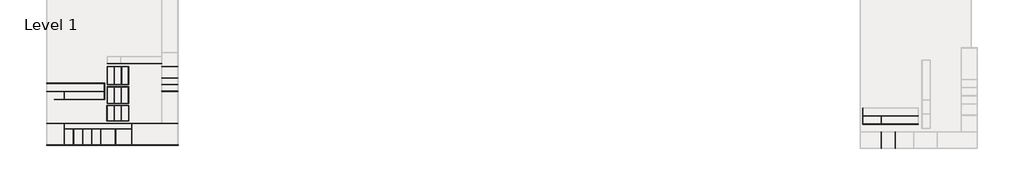
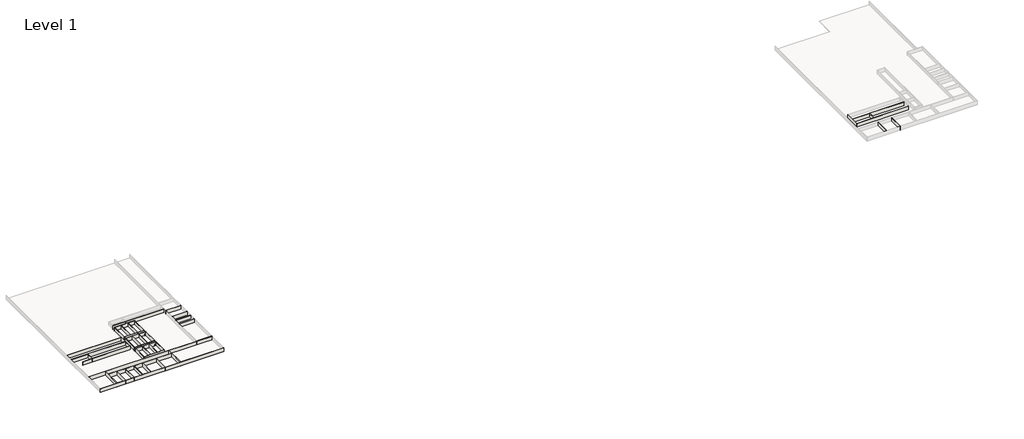
# One storey, part 1 of 4: 45 walls, 12 doors.
# Revit data of these elements (continued)
# Room at (1606634.071, 111947.24) mm, phase "New Construction", upper level "Level 1", upper offset 10.00 ft, lower offset 0.00 ft (continued)
#   Name = "STORAGE"
# Room at (1599894.048, 116775.918) mm, phase "New Construction", upper level "Level 1", upper offset 10.00 ft, lower offset 0.00 ft
#   Number = "64"
#   Name = "Room"
# Room at (1649995.832, 63944.956) mm, phase "New Construction", upper level "Level 1", upper offset 10.00 ft, lower offset 0.00 ft
#   Number = "65"
#   Name = "CLASSROOM"
# Room, not placed, phase "New Construction", upper offset 0.00 ft, lower offset 0.00 ft
#   Number = "165"
#   Name = "RETAIL"
# Room, not placed, phase "New Construction", upper offset 0.00 ft, lower offset 0.00 ft
#   Number = "166"
#   Name = "KITCHEN/CONCESSIONS"
# Room, not placed, phase "New Construction", upper offset 0.00 ft, lower offset 0.00 ft
#   Number = "167"
#   Name = "RETAIL"
# Room, not placed, phase "New Construction", upper offset 0.00 ft, lower offset 0.00 ft
#   Number = "168"
#   Name = "RETAIL"
# Room, not placed, phase "New Construction", upper offset 0.00 ft, lower offset 0.00 ft
#   Number = "169"
#   Name = "XCEL ENTRANCE/LOBBY"
# Room, not placed, phase "New Construction", upper offset 0.00 ft, lower offset 0.00 ft
#   Number = "170"
#   Name = "CLINIC"
# Room, not placed, phase "New Construction", upper offset 0.00 ft, lower offset 0.00 ft
#   Number = "171"
#   Name = "Clinic"
# Room, not placed, phase "New Construction", upper offset 0.00 ft, lower offset 0.00 ft
#   Number = "172"
#   Name = "Room"
# Room, not placed, phase "New Construction", upper offset 0.00 ft, lower offset 0.00 ft
#   Number = "173"
#   Name = "RETAIL"
# Room, not placed, phase "New Construction", upper offset 0.00 ft, lower offset 0.00 ft
#   Number = "174"
#   Name = "RETAIL"
# Room, not placed, phase "New Construction", upper offset 0.00 ft, lower offset 0.00 ft
#   Number = "175"
#   Name = "RETAIL"
# Room, not placed, phase "New Construction", upper offset 0.00 ft, lower offset 0.00 ft
#   Number = "176"
#   Name = "RETAIL"
# Room, not placed, phase "New Construction", upper offset 0.00 ft, lower offset 0.00 ft
#   Number = "177"
#   Name = "Room"
# Room, not placed, phase "New Construction", upper offset 0.00 ft, lower offset 0.00 ft
#   Number = "178"
#   Name = "FLEX SPACE"
# Room, not placed, phase "New Construction", upper offset 0.00 ft, lower offset 0.00 ft
#   Number = "179"
#   Name = "FLEX SPACE"
# Room, not placed, phase "New Construction", upper offset 0.00 ft, lower offset 0.00 ft
#   Number = "180"
#   Name = "FLEX SPACE"
# Room, not placed, phase "New Construction", upper offset 0.00 ft, lower offset 0.00 ft
#   Number = "181"
#   Name = "FLEX SPACE"
# Room, not placed, phase "New Construction", upper offset 0.00 ft, lower offset 0.00 ft
#   Number = "182"
#   Name = "FLEX SPACE"
# Room, not placed, phase "New Construction", upper offset 0.00 ft, lower offset 0.00 ft
#   Number = "183"
#   Name = "FLEX SPACE"
# Room, not placed, phase "New Construction", upper offset 0.00 ft, lower offset 0.00 ft
#   Number = "184"
#   Name = "FLEX SPACE"
# Room, not placed, phase "New Construction", upper offset 0.00 ft, lower offset 0.00 ft
#   Number = "185"
#   Name = "FLEX SPACE"
# Room, not placed, phase "New Construction", upper offset 0.00 ft, lower offset 0.00 ft
#   Number = "186"
#   Name = "RETAIL"
# Room, not placed, phase "New Construction", upper offset 0.00 ft, lower offset 0.00 ft
#   Number = "187"
#   Name = "RETAIL"
# Room, not placed, phase "New Construction", upper offset 0.00 ft, lower offset 0.00 ft
#   Number = "188"
#   Name = "RETAIL"
# Room at (703794.505, -89081.89) mm, phase "New Construction", upper level "Level 1", upper offset 10.00 ft, lower offset 0.00 ft
#   Number = "66"
#   Name = "Clinic"
# Room, not placed, phase "New Construction", upper offset 0.00 ft, lower offset 0.00 ft
#   Number = "133"
#   Name = "CLASSROOM"
# Room at (1599423.332, 28056.316) mm, phase "New Construction", upper level "Level 1", upper offset 10.00 ft, lower offset 0.00 ft
#   Number = "67"
#   Name = "The Alley / Fitness / Free  Weights"
# Room at (671925.982, -22494.563) mm, phase "New Construction", upper level "Level 1", upper offset 10.00 ft, lower offset 0.00 ft
#   Number = "68"
#   Name = "Golf"
# Room at (720901.484, -68666.612) mm, phase "New Construction", upper level "Level 1", upper offset 10.00 ft, lower offset 0.00 ft
#   Number = "69"
#   Name = "ENTRY/RECEPTION"
# Room at (1649074.907, 55092.939) mm, phase "New Construction", upper level "Level 1", upper offset 10.00 ft, lower offset 0.00 ft
#   Number = "70"
#   Name = "STORAGE"
# Room at (670407.687, -88737.153) mm, phase "New Construction", upper level "Level 1", upper offset 10.00 ft, lower offset 0.00 ft
#   Number = "71"
#   Name = "FITNESS CENTER"
# Room at (647282.948, -88737.153) mm, phase "New Construction", upper level "Level 1", upper offset 10.00 ft, lower offset 0.00 ft
#   Number = "72"
#   Name = "KITCHEN"
# Room at (628829.874, -88737.153) mm, phase "New Construction", upper level "Level 1", upper offset 10.00 ft, lower offset 0.00 ft
#   Number = "73"
#   Name = "PIZZA"
# Room at (610376.799, -88737.153) mm, phase "New Construction", upper level "Level 1", upper offset 10.00 ft, lower offset 0.00 ft
#   Number = "74"
#   Name = "SPORTING GOODS"
# Room at (718778.3, -52027.588) mm, phase "New Construction", upper level "Level 1", upper offset 10.00 ft, lower offset 0.00 ft
#   Number = "75"
#   Name = "KITCHEN/CONCESSIONS"
# Room at (720911.9, -42684.259) mm, phase "New Construction", upper level "Level 1", upper offset 10.00 ft, lower offset 0.00 ft
#   Number = "76"
#   Name = "LOCKER ROOM"
# Room at (720911.9, -33504.306) mm, phase "New Construction", upper level "Level 1", upper offset 10.00 ft, lower offset 0.00 ft
#   Number = "77"
#   Name = "LOCKE ROOM"
# Room at (720911.9, -25026.427) mm, phase "New Construction", upper level "Level 1", upper offset 10.00 ft, lower offset 0.00 ft
#   Number = "78"
#   Name = "STORAGE"
# Room at (720911.9, -3102.291) mm, phase "New Construction", upper level "Level 1", upper offset 10.00 ft, lower offset 0.00 ft
#   Number = "79"
#   Name = "EXCEL LOCKER ROOMS"
# Room at (639969.564, -66228.212) mm, phase "New Construction", upper level "Level 1", upper offset 10.00 ft, lower offset 0.00 ft
#   Number = "80"
#   Name = "Fitness"
# Room at (610376.799, -66228.212) mm, phase "New Construction", upper level "Level 1", upper offset 10.00 ft, lower offset 0.00 ft
#   Number = "81"
#   Name = "Storage"
# Room at (627252.746, -56297.723) mm, phase "New Construction", upper level "Level 1", upper offset 10.00 ft, lower offset 0.00 ft
#   Number = "82"
#   Name = "The Alley"
# Room at (635596.434, 33202.417) mm, phase "New Construction", upper level "Level 1", upper offset 10.00 ft, lower offset 0.00 ft
#   Number = "83"
#   Name = "FOOTBALL FIELD"
# Room at (1626848.534, -62440.572) mm, phase "New Construction", upper level "Level 1", upper offset 10.00 ft, lower offset 0.00 ft
#   Number = "84"
#   Name = "PAIN MANAGEMENT"
# Room at (1600357.704, -62440.572) mm, phase "New Construction", upper level "Level 1", upper offset 10.00 ft, lower offset 0.00 ft
#   Number = "85"
#   Name = "DENTAL / CLINIC"
# Room at (1577576.782, -62440.572) mm, phase "New Construction", upper level "Level 1", upper offset 10.00 ft, lower offset 0.00 ft
#   Number = "86"
#   Name = "SUBWAY"
# Room at (1557960.755, -62440.572) mm, phase "New Construction", upper level "Level 1", upper offset 10.00 ft, lower offset 0.00 ft
#   Number = "87"
#   Name = "PIZZA"
# Room at (1536954.616, -62440.572) mm, phase "New Construction", upper level "Level 1", upper offset 10.00 ft, lower offset 0.00 ft
#   Number = "88"
#   Name = "SPORTING GOODS"
# Room at (1564292.975, 28021.565) mm, phase "New Construction", upper level "Level 1", upper offset 10.00 ft, lower offset 0.00 ft
#   Number = "89"
#   Name = "FOOTBALL FIELD"
# Room at (-178341.391, -40050.292) mm, phase "New Construction", upper level "Level 1", upper offset 10.00 ft, lower offset 0.00 ft
#   Number = "190"
#   Name = "FITNESS CENTER"
# Room at (-178021.927, -29963.518) mm, phase "New Construction", upper level "Level 1", upper offset 10.00 ft, lower offset 0.00 ft
#   Number = "220"
#   Name = "LOCKER ROOM"
# Room at (-178021.927, -22815.02) mm, phase "New Construction", upper level "Level 1", upper offset 10.00 ft, lower offset 0.00 ft
#   Number = "221"
#   Name = "LOCKER ROOM"
# Room at (-282117.148, -88776.087) mm, phase "New Construction", upper level "Level 1", upper offset 10.00 ft, lower offset 0.00 ft
#   Number = "193"
#   Name = "PIZZA"
# Room at (-270841.388, -88776.087) mm, phase "New Construction", upper level "Level 1", upper offset 10.00 ft, lower offset 0.00 ft
#   Number = "194"
#   Name = "STARBUCKS"
# Room at (-260384.073, -89114.535) mm, phase "New Construction", upper level "Level 1", upper offset 10.00 ft, lower offset 0.00 ft
#   Number = "195"
#   Name = "SALON"
# Room at (-247403.587, -88717.226) mm, phase "New Construction", upper level "Level 1", upper offset 10.00 ft, lower offset 0.00 ft
#   Number = "196"
#   Name = "DENTIST"
# Room at (-230288.681, -88776.087) mm, phase "New Construction", upper level "Level 1", upper offset 10.00 ft, lower offset 0.00 ft
#   Number = "197"
#   Name = "PAIN MGMT"
# Room at (-244817.251, -9550.032) mm, phase "New Construction", upper level "Level 1", upper offset 10.00 ft, lower offset 0.00 ft
#   Number = "198"
#   Name = "CLASS ROOM"
# Room, not placed, phase "New Construction", upper offset 0.00 ft, lower offset 0.00 ft
#   Number = "199"
#   Name = "CLASS ROOM"
# Room at (-233854.618, -20357.649) mm, phase "New Construction", upper level "Level 1", upper offset 10.00 ft, lower offset 0.00 ft
#   Number = "200"
#   Name = "CLASS ROOM"
# Room, not placed, phase "New Construction", upper offset 0.00 ft, lower offset 0.00 ft
#   Number = "201"
#   Name = "CLASS ROOM"
# Room, not placed, phase "New Construction", upper offset 0.00 ft, lower offset 0.00 ft
#   Number = "202"
#   Name = "CLASS ROOM"
# Room, not placed, phase "New Construction", upper offset 0.00 ft, lower offset 0.00 ft
#   Number = "203"
#   Name = "CLASS ROOM"
# Room at (-238486.151, -32448.015) mm, phase "New Construction", upper level "Level 1", upper offset 10.00 ft, lower offset 0.00 ft
#   Number = "204"
#   Name = "CLASS ROOM"
# Room at (-246553.184, -43328.883) mm, phase "New Construction", upper level "Level 1", upper offset 10.00 ft, lower offset 0.00 ft
#   Number = "205"
#   Name = "CLASS ROOM"
# Room at (-240329.784, -54004.958) mm, phase "New Construction", upper level "Level 1", upper offset 10.00 ft, lower offset 0.00 ft
#   Number = "206"
#   Name = "CLASS ROOM"
# Room, not placed, phase "New Construction", upper offset 0.00 ft, lower offset 0.00 ft
#   Number = "207"
#   Name = "CLASS ROOM"
# Room, not placed, phase "New Construction", upper offset 0.00 ft, lower offset 0.00 ft
#   Number = "208"
#   Name = "STORAGE"
# Room, not placed, phase "New Construction", upper offset 0.00 ft, lower offset 0.00 ft
#   Number = "210"
#   Name = "FITNESS CENTER"
# Room at (-178145.253, -13837.189) mm, phase "New Construction", upper level "Level 1", upper offset 10.00 ft, lower offset 0.00 ft
#   Number = "211"
#   Name = "KITCHEN"
# Room at (-178145.253, 16320.164) mm, phase "New Construction", upper level "Level 1", upper offset 10.00 ft, lower offset 0.00 ft
#   Number = "212"
#   Name = "OFFICES/CONF."
# Room at (-178134.837, 30113.212) mm, phase "New Construction", upper level "Level 1", upper offset 10.00 ft, lower offset 0.00 ft
#   Number = "213"
#   Name = "CLASSROOM"
# Room, not placed, phase "New Construction", upper offset 0.00 ft, lower offset 0.00 ft
#   Number = "209"
#   Name = "STORAGE"
# Room at (672322.647, -64446.408) mm, phase "New Construction", upper level "Level 1", upper offset 10.00 ft, lower offset 0.00 ft
#   Number = "91"
#   Name = "CLASSROOM"
# Room, not placed, phase "New Construction", upper offset 0.00 ft, lower offset 0.00 ft
#   Number = "92"
#   Name = "CLASSROOM"
# Room, not placed, phase "New Construction", upper offset 0.00 ft, lower offset 0.00 ft
#   Number = "2"
#   Name = "Room"
# Room, not placed, phase "New Construction", upper offset 0.00 ft, lower offset 0.00 ft
#   Number = "5"
#   Name = "Room"
# Room, not placed, phase "New Construction", upper offset 0.00 ft, lower offset 0.00 ft
#   Number = "8"
#   Name = "Room"
# Room, not placed, phase "New Construction", upper offset 0.00 ft, lower offset 0.00 ft
#   Number = "9"
#   Name = "Room"
# Room, not placed, phase "New Construction", upper offset 0.00 ft, lower offset 0.00 ft
#   Number = "10"
#   Name = "Clinic"
# Room, not placed, phase "New Construction", upper offset 0.00 ft, lower offset 0.00 ft
#   Number = "14"
#   Name = "Room"
# Room, not placed, phase "New Construction", upper offset 0.00 ft, lower offset 0.00 ft
#   Number = "15"
#   Name = "Room"
# Room, not placed, phase "New Construction", upper offset 0.00 ft, lower offset 0.00 ft
#   Number = "16"
#   Name = "Room"
# Room, not placed, phase "New Construction", upper offset 0.00 ft, lower offset 0.00 ft
#   Number = "17"
#   Name = "Room"
# Room, not placed, phase "New Construction", upper offset 0.00 ft, lower offset 0.00 ft
#   Number = "18"
#   Name = "Room"
# Room, not placed, phase "New Construction", upper offset 0.00 ft, lower offset 0.00 ft
#   Number = "19"
#   Name = "Room"
# Room, not placed, phase "New Construction", upper offset 0.00 ft, lower offset 0.00 ft
#   Number = "21"
#   Name = "Room"
# Room, not placed, phase "New Construction", upper offset 0.00 ft, lower offset 0.00 ft
#   Number = "22"
#   Name = "Room"
# Room, not placed, phase "New Construction", upper offset 0.00 ft, lower offset 0.00 ft
#   Number = "23"
#   Name = "Room"
# Room, not placed, phase "New Construction", upper offset 0.00 ft, lower offset 0.00 ft
#   Number = "24"
#   Name = "Room"
# Room, not placed, phase "New Construction", upper offset 0.00 ft, lower offset 0.00 ft
#   Number = "25"
#   Name = "Room"
# Room, not placed, phase "New Construction", upper offset 0.00 ft, lower offset 0.00 ft
#   Number = "29"
#   Name = "Room"
# Room, not placed, phase "New Construction", upper offset 0.00 ft, lower offset 0.00 ft
#   Number = "32"
#   Name = "Room"
# Room at (-241485.229, 1411.75) mm, phase "New Construction", upper level "Level 1", upper offset 10.00 ft, lower offset 0.00 ft
#   Number = "215"
#   Name = "STORAGE"
# Room at (670326.663, -55930.702) mm, phase "New Construction", upper level "Level 1", upper offset 10.00 ft, lower offset 0.00 ft
#   Number = "96"
#   Name = "CLASSROOM"
# Room at (-175097.296, 94708.366) mm, phase "New Construction", upper level "Level 1", upper offset 10.00 ft, lower offset 0.00 ft
#   Number = "117"
#   Name = "STORAGE/MECH."
# Room, not placed, phase "New Construction", upper offset 0.00 ft, lower offset 0.00 ft
#   Number = "118"
#   Name = "OFFICES/CONF."
# Room, not placed, phase "New Construction", upper offset 0.00 ft, lower offset 0.00 ft
#   Number = "119"
#   Name = "LOCKEROOM"
# Room, not placed, phase "New Construction", upper offset 0.00 ft, lower offset 0.00 ft
#   Number = "120"
#   Name = "KITCHEN/CONCESSIONS"
# Room at (-180671.025, 5671.603) mm, phase "New Construction", upper level "Level 1", upper offset 10.00 ft, lower offset 0.00 ft
#   Number = "121"
#   Name = "ENTRY/RECEPTION"
# Room, not placed, phase "New Construction", upper offset 0.00 ft, lower offset 0.00 ft
#   Number = "122"
#   Name = "CLINIC"
# Room, not placed, phase "New Construction", upper offset 0.00 ft, lower offset 0.00 ft
#   Number = "123"
#   Name = "CLASSROOM"
# Room, not placed, phase "New Construction", upper offset 0.00 ft, lower offset 0.00 ft
#   Number = "124"
#   Name = "CLASSROOM"
# Room, not placed, phase "New Construction", upper offset 0.00 ft, lower offset 0.00 ft
#   Number = "125"
#   Name = "CLASSROOM/SPINNING"
# Room at (-292404.606, -88774.747) mm, phase "New Construction", upper level "Level 1", upper offset 10.00 ft, lower offset 0.00 ft
#   Number = "126"
#   Name = "SUBWAY"
# Room at (-303674.211, -78111.932) mm, phase "New Construction", upper level "Level 1", upper offset 10.00 ft, lower offset 0.00 ft
#   Number = "127"
#   Name = "SPORTING GOODS"
# Room at (-257385.003, -38023.513) mm, phase "New Construction", upper level "Level 1", upper offset 10.00 ft, lower offset 0.00 ft
#   Number = "128"
#   Name = "FITNESS"
# Room at (-304096.877, -38023.513) mm, phase "New Construction", upper level "Level 1", upper offset 10.00 ft, lower offset 0.00 ft
#   Number = "129"
#   Name = "STOR./MECH."
# Room at (-282267.022, -30030.186) mm, phase "New Construction", upper level "Level 1", upper offset 10.00 ft, lower offset 0.00 ft
#   Number = "130"
#   Name = "THE ALLEY"
# Room at (-217895.5, 1411.75) mm, phase "New Construction", upper level "Level 1", upper offset 10.00 ft, lower offset 0.00 ft
#   Number = "131"
#   Name = "GOLF"
# Room, not placed, phase "New Construction", upper offset 0.00 ft, lower offset 0.00 ft
#   Number = "132"
#   Name = "CLASSROOM"
# Room at (-180407.217, 46416.121) mm, phase "New Construction", upper level "Level 1", upper offset 10.00 ft, lower offset 0.00 ft
#   Number = "134"
#   Name = "FITNESS"
# Room, not placed, phase "New Construction", upper offset 0.00 ft, lower offset 0.00 ft
#   Number = "135"
#   Name = "AEROBICS/YOGA"
# Room, not placed, phase "New Construction", upper offset 0.00 ft, lower offset 0.00 ft
#   Number = "136"
#   Name = "CLASSROOM"
# Room, not placed, phase "New Construction", upper offset 0.00 ft, lower offset 0.00 ft
#   Number = "33"
#   Name = "Room"
# Room, not placed, phase "New Construction", upper offset 0.00 ft, lower offset 0.00 ft
#   Number = "34"
#   Name = "Room"
# Room, not placed, phase "New Construction", upper offset 0.00 ft, lower offset 0.00 ft
#   Number = "35"
#   Name = "Room"
# Room, not placed, phase "New Construction", upper offset 0.00 ft, lower offset 0.00 ft
#   Number = "36"
#   Name = "Room"
# Room, not placed, phase "New Construction", upper offset 0.00 ft, lower offset 0.00 ft
#   Number = "37"
#   Name = "Room"
# Room, not placed, phase "New Construction", upper offset 0.00 ft, lower offset 0.00 ft
#   Number = "38"
#   Name = "Room"
# Room, not placed, phase "New Construction", upper offset 0.00 ft, lower offset 0.00 ft
#   Number = "39"
#   Name = "Clinic"
# Room, not placed, phase "New Construction", upper offset 0.00 ft, lower offset 0.00 ft
#   Number = "40"
#   Name = "Room"
# Room, not placed, phase "New Construction", upper offset 0.00 ft, lower offset 0.00 ft
#   Number = "41"
#   Name = "Room"
# Room, not placed, phase "New Construction", upper offset 0.00 ft, lower offset 0.00 ft
#   Number = "42"
#   Name = "Room"
# Room, not placed, phase "New Construction", upper offset 0.00 ft, lower offset 0.00 ft
#   Number = "43"
#   Name = "Room"
# Room, not placed, phase "New Construction", upper offset 0.00 ft, lower offset 0.00 ft
#   Number = "44"
#   Name = "Room"
# Room, not placed, phase "New Construction", upper offset 0.00 ft, lower offset 0.00 ft
#   Number = "45"
#   Name = "Fitness"
# Room, not placed, phase "New Construction", upper offset 0.00 ft, lower offset 0.00 ft
#   Number = "46"
#   Name = "Storage"
# Room, not placed, phase "New Construction", upper offset 0.00 ft, lower offset 0.00 ft
#   Number = "47"
#   Name = "The Alley"
# Room at (-228742.742, -34392.285) mm, phase "New Construction", upper level "Level 1", upper offset 10.00 ft, lower offset 0.00 ft
#   Number = "216"
#   Name = "CLASS ROOM"
# Room, not placed, phase "New Construction", upper offset 0.00 ft, lower offset 0.00 ft
#   Number = "137"
#   Name = "CLASSROOM"
# Room at (-228742.742, -11392.397) mm, phase "New Construction", upper level "Level 1", upper offset 10.00 ft, lower offset 0.00 ft
#   Number = "217"
#   Name = "CLASS ROOM"
# Room at (-228742.742, -55897.452) mm, phase "New Construction", upper level "Level 1", upper offset 10.00 ft, lower offset 0.00 ft
#   Number = "218"
#   Name = "CLASS ROOM"
# Room at (-244685.532, -55897.452) mm, phase "New Construction", upper level "Level 1", upper offset 10.00 ft, lower offset 0.00 ft
#   Number = "219"
#   Name = "CLASS ROOM"
# Room at (1588361.539, 84512.004) mm, phase "New Construction", upper level "Level 1", upper offset 10.00 ft, lower offset 0.00 ft
#   Number = "90"
#   Name = "Room"
# Room at (2460506.754, -35163.043) mm, phase "New Construction", upper level "Level 1", upper offset 10.00 ft, lower offset 0.00 ft
#   Number = "138"
#   Name = "CLINIC"
# Room at (-264121.563, -73054.927) mm, phase "New Construction", upper level "Level 1", upper offset 10.00 ft, lower offset 0.00 ft
#   Number = "214"
#   Name = "HALLWAY / FLEX SPACE"
# Room at (2488320.402, -35163.043) mm, phase "New Construction", upper level "Level 1", upper offset 10.00 ft, lower offset 0.00 ft
#   Number = "139"
#   Name = "KITCHEN/CONCESSIONS"
# Room at (2504050.059, -35163.043) mm, phase "New Construction", upper level "Level 1", upper offset 10.00 ft, lower offset 0.00 ft
#   Number = "140"
#   Name = "XCEL ENTRANCE"
# Room at (2522624.517, -33639.043) mm, phase "New Construction", upper level "Level 1", upper offset 10.00 ft, lower offset 0.00 ft
#   Number = "141"
#   Name = "LOCKER ROOM"
# Room at (2543990.806, -35163.043) mm, phase "New Construction", upper level "Level 1", upper offset 10.00 ft, lower offset 0.00 ft
#   Number = "142"
#   Name = "RETAIL"
# Room at (2569660.809, -35163.043) mm, phase "New Construction", upper level "Level 1", upper offset 10.00 ft, lower offset 0.00 ft
#   Number = "143"
#   Name = "RETAIL"
# Room at (2589948.392, -35163.043) mm, phase "New Construction", upper level "Level 1", upper offset 10.00 ft, lower offset 0.00 ft
#   Number = "144"
#   Name = "RETAIL"
# Room at (2605324.829, -28341.246) mm, phase "New Construction", upper level "Level 1", upper offset 10.00 ft, lower offset 0.00 ft
#   Number = "145"
#   Name = "RETAIL"
# Room at (2605324.829, -1636.162) mm, phase "New Construction", upper level "Level 1", upper offset 10.00 ft, lower offset 0.00 ft
#   Number = "146"
#   Name = "RETAIL"
# Room at (2605324.829, 21963.679) mm, phase "New Construction", upper level "Level 1", upper offset 10.00 ft, lower offset 0.00 ft
#   Number = "147"
#   Name = "RETAIL"
# Room at (2605324.829, 48047.714) mm, phase "New Construction", upper level "Level 1", upper offset 10.00 ft, lower offset 0.00 ft
#   Number = "148"
#   Name = "RETAIL"
# Room at (2605324.829, 67248.226) mm, phase "New Construction", upper level "Level 1", upper offset 10.00 ft, lower offset 0.00 ft
#   Number = "149"
#   Name = "RETAIL"
# Room at (-191516.975, -85535.682) mm, phase "New Construction", upper level "Level 1", upper offset 10.00 ft, lower offset 0.00 ft
#   Number = "189"
#   Name = "CLINIC"
# Room at (2522593.022, -35170.673) mm, phase "New Construction", upper level "Level 1", upper offset 10.00 ft, lower offset 0.00 ft
#   Number = "150"
#   Name = "LOCKER ROOM"
